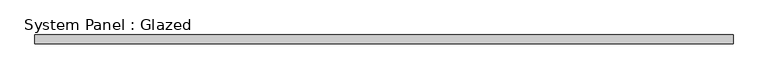
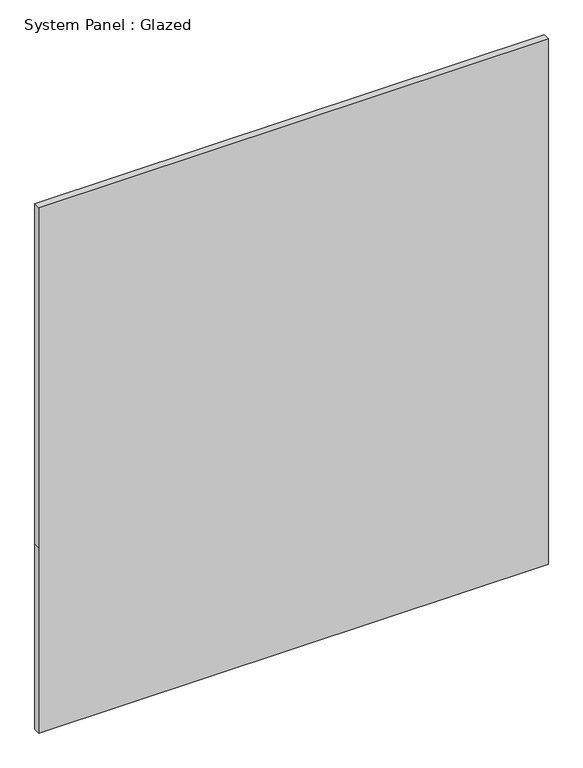
"""IFC4 building model written with IfcOpenShell, lengths in millimetres: plate geometry, System Panel : Glazed."""

import ifcopenshell
import ifcopenshell.guid

model = None  # the IFC model being written
_history = None  # IfcOwnerHistory: only IFC2X3 demands one
_inside = {}  # id of a spatial element -> (the spatial element, [elements in it])
_under = {}  # id of a project, library or spatial element -> (it, [spatial elements below it])
_declared = {}  # id of a project -> (the project, [libraries it declares])
_typed = {}  # id of a type object -> (the type object, [elements of that type])
_made_of = {}  # id of a material, layer set ... -> (it, [elements and type objects made of it])


def new_model(schema):
    """Start an empty IFC model of exactly this schema.

    Asked for "IFC4X3", IfcOpenShell would pick the latest addendum, in which some entities
    have other attributes; the version numbers below select the first issue.
    IFC2X3 requires an IfcOwnerHistory on every rooted entity: one is made here for all.
    """
    global model, _history
    if schema == "IFC4X3":
        model = ifcopenshell.file(schema_version=(4, 3, 0, 0))
    else:
        model = ifcopenshell.file(schema=schema)
    _inside.clear()
    _under.clear()
    _declared.clear()
    _typed.clear()
    _made_of.clear()
    _history = None
    if model.schema == "IFC2X3":
        org = make("IfcOrganization", Name="unknown")
        user = make(
            "IfcPersonAndOrganization",
            ThePerson=make("IfcPerson", FamilyName="unknown"),
            TheOrganization=org,
        )
        app = make(
            "IfcApplication",
            ApplicationDeveloper=org,
            Version="unknown",
            ApplicationFullName="unknown",
            ApplicationIdentifier="unknown",
        )
        _history = make(
            "IfcOwnerHistory",
            OwningUser=user,
            OwningApplication=app,
            ChangeAction="ADDED",
            CreationDate=0,
        )
    return model


def make(cls, **values):
    """One entity of the class cls with the attributes given. An attribute that is None is left unset."""
    return model.create_entity(
        cls, **{name: value for name, value in values.items() if value is not None}
    )


def rooted(cls, **values):
    """An entity with a GlobalId (a new one), such as an element, a storey or a relation."""
    return make(cls, GlobalId=ifcopenshell.guid.new(), OwnerHistory=_history, **values)


def si_unit(unit_type, name, prefix=None):
    """IfcSIUnit, for example si_unit("LENGTHUNIT", "METRE", prefix="MILLI")."""
    return make("IfcSIUnit", UnitType=unit_type, Prefix=prefix, Name=name)


def assignment(units):
    """IfcUnitAssignment: the units of a project."""
    return None if units is None else make("IfcUnitAssignment", Units=units)


def point(xyz):
    """IfcCartesianPoint."""
    return None if xyz is None else make("IfcCartesianPoint", Coordinates=xyz)


def direction(xyz):
    """IfcDirection."""
    return None if xyz is None else make("IfcDirection", DirectionRatios=xyz)


def frame(location, z_axis=None, x_axis=None):
    """IfcAxis2Placement3D, a coordinate frame: its origin and axes. An axis left out is left unset."""
    return make(
        "IfcAxis2Placement3D",
        Location=point(location),
        Axis=direction(z_axis),
        RefDirection=direction(x_axis),
    )


def origin():
    """The frame at (0, 0, 0) with its axes left unset."""
    return frame((0.0, 0.0, 0.0))


def place(relative_to, where):
    """IfcLocalPlacement: puts the frame where relative to a parent placement (None: the world)."""
    return make(
        "IfcLocalPlacement", PlacementRelTo=relative_to, RelativePlacement=where
    )


def context(
    kind, dimensions, precision=None, world=None, true_north=None, identifier=None
):
    """IfcGeometricRepresentationContext, for example the 3D "Model" context."""
    return make(
        "IfcGeometricRepresentationContext",
        ContextIdentifier=identifier,
        ContextType=kind,
        CoordinateSpaceDimension=dimensions,
        Precision=precision,
        WorldCoordinateSystem=world,
        TrueNorth=true_north,
    )


def project(units=None, contexts=None):
    """IfcProject with its units and contexts."""
    return rooted(
        "IfcProject",
        Name="project",
        RepresentationContexts=contexts,
        UnitsInContext=assignment(units),
    )


def spatial(cls, under=None, at=None, **own):
    """A site, building, storey or space (cls), placed at a placement, below another one or the project."""
    s = rooted(cls, ObjectPlacement=at, **own)
    if under is not None:
        _under.setdefault(under.id(), (under, []))[1].append(s)
    return s


def polyline(points):
    """IfcPolyline through the points."""
    return make("IfcPolyline", Points=[point(p) for p in points])


def outline(outer, holes=None, kind="AREA"):
    """IfcArbitraryClosedProfileDef: a profile drawn as a closed curve; with holes, ...WithVoids."""
    if holes is None:
        return make("IfcArbitraryClosedProfileDef", ProfileType=kind, OuterCurve=outer)
    return make(
        "IfcArbitraryProfileDefWithVoids",
        ProfileType=kind,
        OuterCurve=outer,
        InnerCurves=holes,
    )


def extrude(swept, where, along, depth):
    """IfcExtrudedAreaSolid: the profile swept, set in the frame where, extruded along a direction by depth."""
    return make(
        "IfcExtrudedAreaSolid",
        SweptArea=swept,
        Position=where,
        ExtrudedDirection=direction(along),
        Depth=depth,
    )


def shape(context_of_items, identifier, shape_type, items):
    """IfcShapeRepresentation: the items that make up one representation, for example the "Body"."""
    return make(
        "IfcShapeRepresentation",
        ContextOfItems=context_of_items,
        RepresentationIdentifier=identifier,
        RepresentationType=shape_type,
        Items=items,
    )


def source(mapping_origin, context_of_items, identifier, shape_type, items):
    """IfcRepresentationMap: a shape defined once, which mapped items show again and again."""
    return make(
        "IfcRepresentationMap",
        MappingOrigin=mapping_origin,
        MappedRepresentation=shape(context_of_items, identifier, shape_type, items),
    )


def transform(
    local_origin,
    x_axis=None,
    y_axis=None,
    z_axis=None,
    scale=None,
    scale2=None,
    scale3=None,
    uniform=True,
):
    """IfcCartesianTransformationOperator3D, or its non-uniform kind. x_axis, y_axis, z_axis: its Axis1, 2, 3."""
    if uniform:
        return make(
            "IfcCartesianTransformationOperator3D",
            Axis1=direction(x_axis),
            Axis2=direction(y_axis),
            LocalOrigin=point(local_origin),
            Scale=scale,
            Axis3=direction(z_axis),
        )
    return make(
        "IfcCartesianTransformationOperator3DnonUniform",
        Axis1=direction(x_axis),
        Axis2=direction(y_axis),
        LocalOrigin=point(local_origin),
        Scale=scale,
        Axis3=direction(z_axis),
        Scale2=scale2,
        Scale3=scale3,
    )


def mapped(mapping_source, mapping_target):
    """IfcMappedItem: shows the shape of a source again, moved by a transform."""
    return make(
        "IfcMappedItem", MappingSource=mapping_source, MappingTarget=mapping_target
    )


def made_of(thing, what):
    """Note that an element or type object is made of a material, layer set ...; save() writes the relation."""
    if what is not None:
        _made_of.setdefault(what.id(), (what, []))[1].append(thing)
    return thing


def element(
    cls,
    number,
    at=None,
    inside=None,
    cuts=None,
    type_object=None,
    material=None,
    context=None,
    identifier="Body",
    shape_type=None,
    held_by="IfcProductDefinitionShape",
    body=None,
    shapes=None,
    **own,
):
    """One element of the class cls, such as IfcWall. Its Tag is "e" and its number.

    at: its placement. inside: the storey or other place that contains it. cuts: it is an
    opening in that element (IfcRelVoidsElement). A single representation is given by context,
    identifier, shape_type and body (its items); several are given by shapes. held_by: the class
    of the entity that holds the representations. save() writes the other relations.
    """
    e = rooted(cls, Tag="e%d" % number, ObjectPlacement=at, **own)
    if body is not None:
        shapes = [shape(context, identifier, shape_type, body)]
    if shapes is not None:
        e.Representation = make(held_by, Representations=shapes)
    if inside is not None:
        _inside.setdefault(inside.id(), (inside, []))[1].append(e)
    if cuts is not None:
        rooted(
            "IfcRelVoidsElement", RelatingBuildingElement=cuts, RelatedOpeningElement=e
        )
    if type_object is not None:
        _typed.setdefault(type_object.id(), (type_object, []))[1].append(e)
    return made_of(e, material)


def aggregate(whole, parts):
    """IfcRelAggregates: a whole, such as a stair, and the parts it consists of."""
    return rooted("IfcRelAggregates", RelatingObject=whole, RelatedObjects=parts)


def save(model, path):
    """Write the relations noted so far, then the file.

    IfcRelAggregates (storeys below a building ...), IfcRelContainedInSpatialStructure (elements
    in a storey), IfcRelDefinesByType, IfcRelAssociatesMaterial and IfcRelDeclares: one each for
    every whole, place, type object, material and project.
    """
    for whole, parts in _under.values():
        aggregate(whole, parts)
    for where, things in _inside.values():
        rooted(
            "IfcRelContainedInSpatialStructure",
            RelatedElements=things,
            RelatingStructure=where,
        )
    for kind, things in _typed.values():
        rooted("IfcRelDefinesByType", RelatedObjects=things, RelatingType=kind)
    for what, things in _made_of.values():
        rooted("IfcRelAssociatesMaterial", RelatedObjects=things, RelatingMaterial=what)
    for by, libraries in _declared.values():
        rooted("IfcRelDeclares", RelatingContext=by, RelatedDefinitions=libraries)
    model.write(path)


def system_panel_glazed_1e38db9b(model_context):
    return source(origin(), model_context, "Body", "SweptSolid", [
        extrude(outline(polyline([(0.0, -975.0000002), (0.0, 975.0000002), (750.0, 975.0000002), (2125.0, 975.0000002), (2125.0, -975.0000002), (750.0, -975.0000002), (0.0, -975.0000002)])), frame((0.0, 24.5, 0.0), z_axis=(0.0, 1.0, 0.0), x_axis=(0.0, 0.0, 1.0)), (0.0, 0.0, 1.0), 25.0),
    ])


if __name__ == "__main__":
    model = new_model("IFC4")
    model_context = context("Model", 3, world=origin())
    ifc_project = project(units=[si_unit("LENGTHUNIT", "METRE", prefix="MILLI")], contexts=[model_context])
    site = spatial("IfcSite", under=ifc_project)
    building = spatial("IfcBuilding", under=site)
    placement = place(None, origin())
    system_panel_glazed_shape = system_panel_glazed_1e38db9b(model_context)
    element("IfcPlate", 1, ObjectType="System Panel : Glazed", at=placement, inside=building, context=model_context, shape_type="MappedRepresentation", body=[
        mapped(system_panel_glazed_shape, transform((0.0, 0.0, 0.0), x_axis=(1.0, 0.0, 0.0), y_axis=(0.0, 1.0, 0.0), z_axis=(0.0, 0.0, 1.0))),
    ])
    save(model, "model.ifc")

# Revit data of these elements
# Element 1 (IfcPlate, "System Panel : Glazed")
#   Materials on its faces: "Glass"
# Materials
#   "Glass": class "Glass", colour RGB 0 128 192, transparency 0.9
